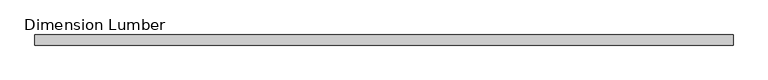
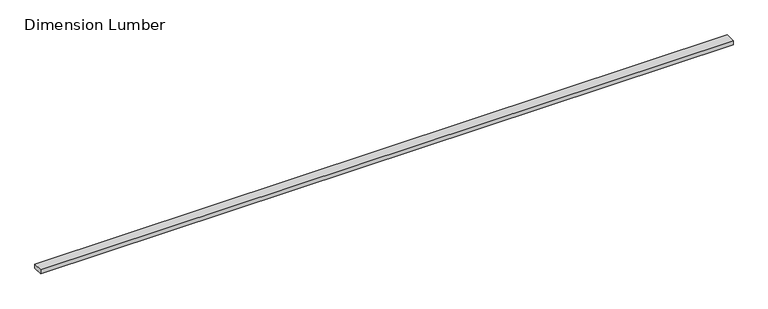
"""IFC4 building model written with IfcOpenShell, lengths in millimetres: beam geometry, Dimension Lumber : Top Supporting Lumbers."""

from ifc_helpers import new_model, si_unit, frame, origin, place, context, project, spatial, polyline, outline, extrude, source, transform, mapped, element, save


def dimension_lumber_f5869125(model_context):
    return source(origin(), model_context, "Body", "SweptSolid", [
        extrude(outline(polyline([(3033.7125, 44.45), (3033.7125, -44.45), (-3116.2625, -44.45), (-3116.2625, 44.45), (3033.7125, 44.45)])), frame((0.0, 0.0, -19.05), z_axis=(0.0, 0.0, 1.0), x_axis=(1.0, 0.0, 0.0)), (0.0, 0.0, 1.0), 38.1),
    ])


if __name__ == "__main__":
    model = new_model("IFC4")
    model_context = context("Model", 3, world=origin())
    ifc_project = project(units=[si_unit("LENGTHUNIT", "METRE", prefix="MILLI")], contexts=[model_context])
    site = spatial("IfcSite", under=ifc_project)
    building = spatial("IfcBuilding", under=site)
    placement = place(None, origin())
    dimension_lumber_shape = dimension_lumber_f5869125(model_context)
    element("IfcBeam", 1, ObjectType="Dimension Lumber : Top Supporting Lumbers", at=placement, inside=building, context=model_context, shape_type="MappedRepresentation", body=[
        mapped(dimension_lumber_shape, transform((0.0, 0.0, 0.0), x_axis=(1.0, 0.0, 0.0), y_axis=(0.0, 1.0, 0.0), z_axis=(0.0, 0.0, 1.0))),
    ])
    save(model, "model.ifc")

# Revit data of these elements
# Type "Dimension Lumber : Top Supporting Lumbers"
#   Assembly Code = "B10"
#   A = 0.0364583 SF
#   Length [instance default] = 5' - 0"
#   b = 0' - 3 1/2"
#   d = 0' - 1 1/2"
#   Structural Material [instance default] = Softwood, Lumber
# Element 1 (IfcBeam, "Dimension Lumber : Top Supporting Lumbers")
#   Structural Material = Douglas Fir #2
#   Materials on its faces: "Douglas Fir #2"
# Materials
#   "Softwood, Lumber": class "Wood", colour RGB 223 192 134, transparency 0, Description = "Pinus Echinata", Cost = 0
#   "Douglas Fir #2": class "Wood", colour RGB 223 192 134, transparency 0, Description = "Pinus Echinata", Cost = 0
